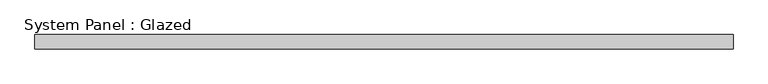
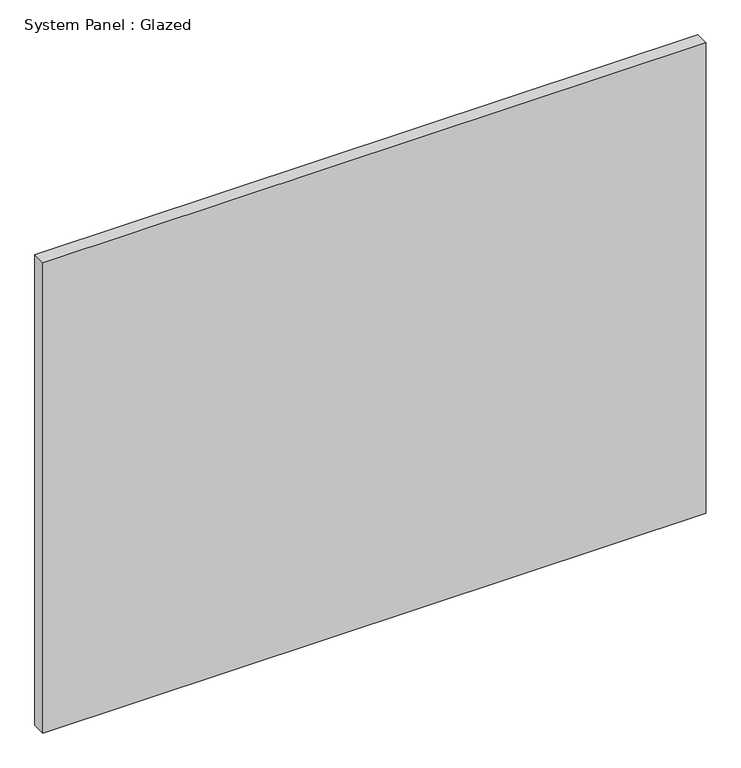
"""IFC4 building model written with IfcOpenShell, lengths in millimetres: plate geometry, System Panel : Glazed."""

import ifcopenshell
import ifcopenshell.guid

model = None  # the IFC model being written
_history = None  # IfcOwnerHistory: only IFC2X3 demands one
_inside = {}  # id of a spatial element -> (the spatial element, [elements in it])
_under = {}  # id of a project, library or spatial element -> (it, [spatial elements below it])
_declared = {}  # id of a project -> (the project, [libraries it declares])
_typed = {}  # id of a type object -> (the type object, [elements of that type])
_made_of = {}  # id of a material, layer set ... -> (it, [elements and type objects made of it])


def new_model(schema):
    """Start an empty IFC model of exactly this schema.

    Asked for "IFC4X3", IfcOpenShell would pick the latest addendum, in which some entities
    have other attributes; the version numbers below select the first issue.
    IFC2X3 requires an IfcOwnerHistory on every rooted entity: one is made here for all.
    """
    global model, _history
    if schema == "IFC4X3":
        model = ifcopenshell.file(schema_version=(4, 3, 0, 0))
    else:
        model = ifcopenshell.file(schema=schema)
    _inside.clear()
    _under.clear()
    _declared.clear()
    _typed.clear()
    _made_of.clear()
    _history = None
    if model.schema == "IFC2X3":
        org = make("IfcOrganization", Name="unknown")
        user = make(
            "IfcPersonAndOrganization",
            ThePerson=make("IfcPerson", FamilyName="unknown"),
            TheOrganization=org,
        )
        app = make(
            "IfcApplication",
            ApplicationDeveloper=org,
            Version="unknown",
            ApplicationFullName="unknown",
            ApplicationIdentifier="unknown",
        )
        _history = make(
            "IfcOwnerHistory",
            OwningUser=user,
            OwningApplication=app,
            ChangeAction="ADDED",
            CreationDate=0,
        )
    return model


def make(cls, **values):
    """One entity of the class cls with the attributes given. An attribute that is None is left unset."""
    return model.create_entity(
        cls, **{name: value for name, value in values.items() if value is not None}
    )


def rooted(cls, **values):
    """An entity with a GlobalId (a new one), such as an element, a storey or a relation."""
    return make(cls, GlobalId=ifcopenshell.guid.new(), OwnerHistory=_history, **values)


def si_unit(unit_type, name, prefix=None):
    """IfcSIUnit, for example si_unit("LENGTHUNIT", "METRE", prefix="MILLI")."""
    return make("IfcSIUnit", UnitType=unit_type, Prefix=prefix, Name=name)


def assignment(units):
    """IfcUnitAssignment: the units of a project."""
    return None if units is None else make("IfcUnitAssignment", Units=units)


def point(xyz):
    """IfcCartesianPoint."""
    return None if xyz is None else make("IfcCartesianPoint", Coordinates=xyz)


def direction(xyz):
    """IfcDirection."""
    return None if xyz is None else make("IfcDirection", DirectionRatios=xyz)


def frame(location, z_axis=None, x_axis=None):
    """IfcAxis2Placement3D, a coordinate frame: its origin and axes. An axis left out is left unset."""
    return make(
        "IfcAxis2Placement3D",
        Location=point(location),
        Axis=direction(z_axis),
        RefDirection=direction(x_axis),
    )


def origin():
    """The frame at (0, 0, 0) with its axes left unset."""
    return frame((0.0, 0.0, 0.0))


def origin_with_axes():
    """The frame at (0, 0, 0) with the z axis (0, 0, 1) and the x axis (1, 0, 0) written out."""
    return frame((0.0, 0.0, 0.0), z_axis=(0.0, 0.0, 1.0), x_axis=(1.0, 0.0, 0.0))


def place(relative_to, where):
    """IfcLocalPlacement: puts the frame where relative to a parent placement (None: the world)."""
    return make(
        "IfcLocalPlacement", PlacementRelTo=relative_to, RelativePlacement=where
    )


def context(
    kind, dimensions, precision=None, world=None, true_north=None, identifier=None
):
    """IfcGeometricRepresentationContext, for example the 3D "Model" context."""
    return make(
        "IfcGeometricRepresentationContext",
        ContextIdentifier=identifier,
        ContextType=kind,
        CoordinateSpaceDimension=dimensions,
        Precision=precision,
        WorldCoordinateSystem=world,
        TrueNorth=true_north,
    )


def project(units=None, contexts=None):
    """IfcProject with its units and contexts."""
    return rooted(
        "IfcProject",
        Name="project",
        RepresentationContexts=contexts,
        UnitsInContext=assignment(units),
    )


def spatial(cls, under=None, at=None, **own):
    """A site, building, storey or space (cls), placed at a placement, below another one or the project."""
    s = rooted(cls, ObjectPlacement=at, **own)
    if under is not None:
        _under.setdefault(under.id(), (under, []))[1].append(s)
    return s


def polyline(points):
    """IfcPolyline through the points."""
    return make("IfcPolyline", Points=[point(p) for p in points])


def outline(outer, holes=None, kind="AREA"):
    """IfcArbitraryClosedProfileDef: a profile drawn as a closed curve; with holes, ...WithVoids."""
    if holes is None:
        return make("IfcArbitraryClosedProfileDef", ProfileType=kind, OuterCurve=outer)
    return make(
        "IfcArbitraryProfileDefWithVoids",
        ProfileType=kind,
        OuterCurve=outer,
        InnerCurves=holes,
    )


def extrude(swept, where, along, depth):
    """IfcExtrudedAreaSolid: the profile swept, set in the frame where, extruded along a direction by depth."""
    return make(
        "IfcExtrudedAreaSolid",
        SweptArea=swept,
        Position=where,
        ExtrudedDirection=direction(along),
        Depth=depth,
    )


def shape(context_of_items, identifier, shape_type, items):
    """IfcShapeRepresentation: the items that make up one representation, for example the "Body"."""
    return make(
        "IfcShapeRepresentation",
        ContextOfItems=context_of_items,
        RepresentationIdentifier=identifier,
        RepresentationType=shape_type,
        Items=items,
    )


def source(mapping_origin, context_of_items, identifier, shape_type, items):
    """IfcRepresentationMap: a shape defined once, which mapped items show again and again."""
    return make(
        "IfcRepresentationMap",
        MappingOrigin=mapping_origin,
        MappedRepresentation=shape(context_of_items, identifier, shape_type, items),
    )


def transform(
    local_origin,
    x_axis=None,
    y_axis=None,
    z_axis=None,
    scale=None,
    scale2=None,
    scale3=None,
    uniform=True,
):
    """IfcCartesianTransformationOperator3D, or its non-uniform kind. x_axis, y_axis, z_axis: its Axis1, 2, 3."""
    if uniform:
        return make(
            "IfcCartesianTransformationOperator3D",
            Axis1=direction(x_axis),
            Axis2=direction(y_axis),
            LocalOrigin=point(local_origin),
            Scale=scale,
            Axis3=direction(z_axis),
        )
    return make(
        "IfcCartesianTransformationOperator3DnonUniform",
        Axis1=direction(x_axis),
        Axis2=direction(y_axis),
        LocalOrigin=point(local_origin),
        Scale=scale,
        Axis3=direction(z_axis),
        Scale2=scale2,
        Scale3=scale3,
    )


def mapped(mapping_source, mapping_target):
    """IfcMappedItem: shows the shape of a source again, moved by a transform."""
    return make(
        "IfcMappedItem", MappingSource=mapping_source, MappingTarget=mapping_target
    )


def made_of(thing, what):
    """Note that an element or type object is made of a material, layer set ...; save() writes the relation."""
    if what is not None:
        _made_of.setdefault(what.id(), (what, []))[1].append(thing)
    return thing


def element(
    cls,
    number,
    at=None,
    inside=None,
    cuts=None,
    type_object=None,
    material=None,
    context=None,
    identifier="Body",
    shape_type=None,
    held_by="IfcProductDefinitionShape",
    body=None,
    shapes=None,
    **own,
):
    """One element of the class cls, such as IfcWall. Its Tag is "e" and its number.

    at: its placement. inside: the storey or other place that contains it. cuts: it is an
    opening in that element (IfcRelVoidsElement). A single representation is given by context,
    identifier, shape_type and body (its items); several are given by shapes. held_by: the class
    of the entity that holds the representations. save() writes the other relations.
    """
    e = rooted(cls, Tag="e%d" % number, ObjectPlacement=at, **own)
    if body is not None:
        shapes = [shape(context, identifier, shape_type, body)]
    if shapes is not None:
        e.Representation = make(held_by, Representations=shapes)
    if inside is not None:
        _inside.setdefault(inside.id(), (inside, []))[1].append(e)
    if cuts is not None:
        rooted(
            "IfcRelVoidsElement", RelatingBuildingElement=cuts, RelatedOpeningElement=e
        )
    if type_object is not None:
        _typed.setdefault(type_object.id(), (type_object, []))[1].append(e)
    return made_of(e, material)


def aggregate(whole, parts):
    """IfcRelAggregates: a whole, such as a stair, and the parts it consists of."""
    return rooted("IfcRelAggregates", RelatingObject=whole, RelatedObjects=parts)


def save(model, path):
    """Write the relations noted so far, then the file.

    IfcRelAggregates (storeys below a building ...), IfcRelContainedInSpatialStructure (elements
    in a storey), IfcRelDefinesByType, IfcRelAssociatesMaterial and IfcRelDeclares: one each for
    every whole, place, type object, material and project.
    """
    for whole, parts in _under.values():
        aggregate(whole, parts)
    for where, things in _inside.values():
        rooted(
            "IfcRelContainedInSpatialStructure",
            RelatedElements=things,
            RelatingStructure=where,
        )
    for kind, things in _typed.values():
        rooted("IfcRelDefinesByType", RelatedObjects=things, RelatingType=kind)
    for what, things in _made_of.values():
        rooted("IfcRelAssociatesMaterial", RelatedObjects=things, RelatingMaterial=what)
    for by, libraries in _declared.values():
        rooted("IfcRelDeclares", RelatingContext=by, RelatedDefinitions=libraries)
    model.write(path)


def system_panel_glazed_8b63b301(model_context):
    return source(origin(), model_context, "Body", "SweptSolid", [
        extrude(outline(polyline([(609.6, 19.05), (-609.6, 19.05), (-609.6, 44.45), (609.6, 44.45), (609.6, 19.05)])), origin_with_axes(), (0.0, 0.0, 1.0), 914.4),
    ])


if __name__ == "__main__":
    model = new_model("IFC4")
    model_context = context("Model", 3, world=origin())
    ifc_project = project(units=[si_unit("LENGTHUNIT", "METRE", prefix="MILLI")], contexts=[model_context])
    site = spatial("IfcSite", under=ifc_project)
    building = spatial("IfcBuilding", under=site)
    placement = place(None, origin())
    system_panel_glazed_shape = system_panel_glazed_8b63b301(model_context)
    element("IfcPlate", 1, ObjectType="System Panel : Glazed", at=placement, inside=building, context=model_context, shape_type="MappedRepresentation", body=[
        mapped(system_panel_glazed_shape, transform((0.0, 0.0, 0.0), x_axis=(1.0, 0.0, 0.0), y_axis=(0.0, 1.0, 0.0), z_axis=(0.0, 0.0, 1.0))),
    ])
    save(model, "model.ifc")

# Revit data of these elements
# Type "System Panel : Glazed"
#   Construction Type Id = "GSP4R"
#   Analytic Construction = "1/8 in Pilkington single glazing"
#   Visual Light Transmittance = 0.9
#   Solar Heat Gain Coefficient = 0.86
#   Heat Transfer Coefficient (U) = 1.18115 BTU/(h·ft²·°F)
#   Define Thermal Properties by = 1
# Element 1 (IfcPlate, "System Panel : Glazed")
#   Materials on its faces: "Glass"
# Materials
#   "Glass": class "Glass", colour RGB 0 128 192, transparency 0.75, Description = "Soda Lime Glass", Cost = 0
